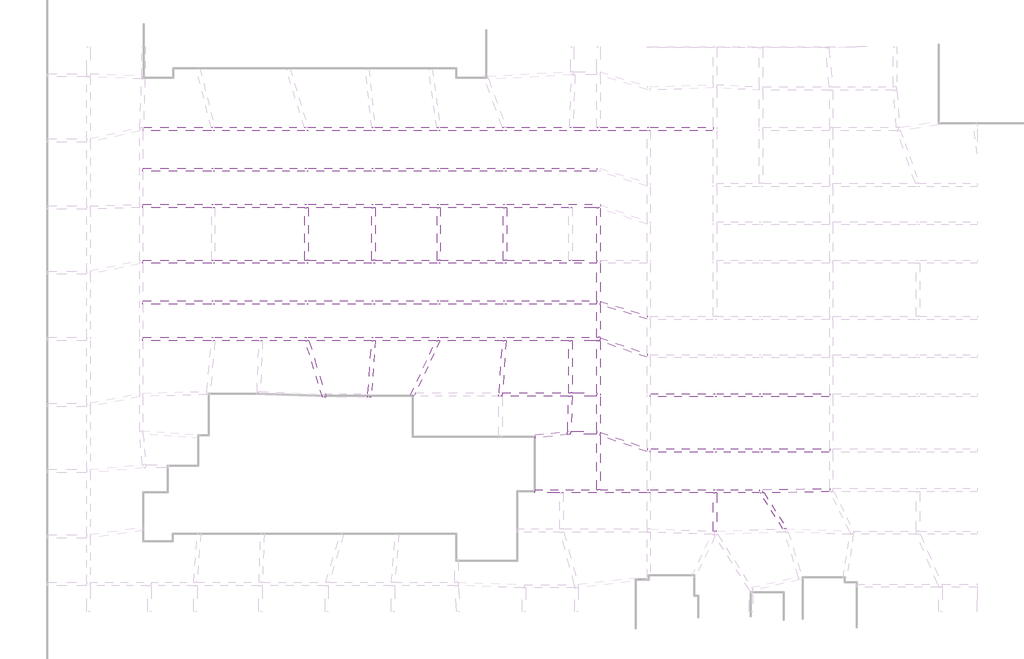
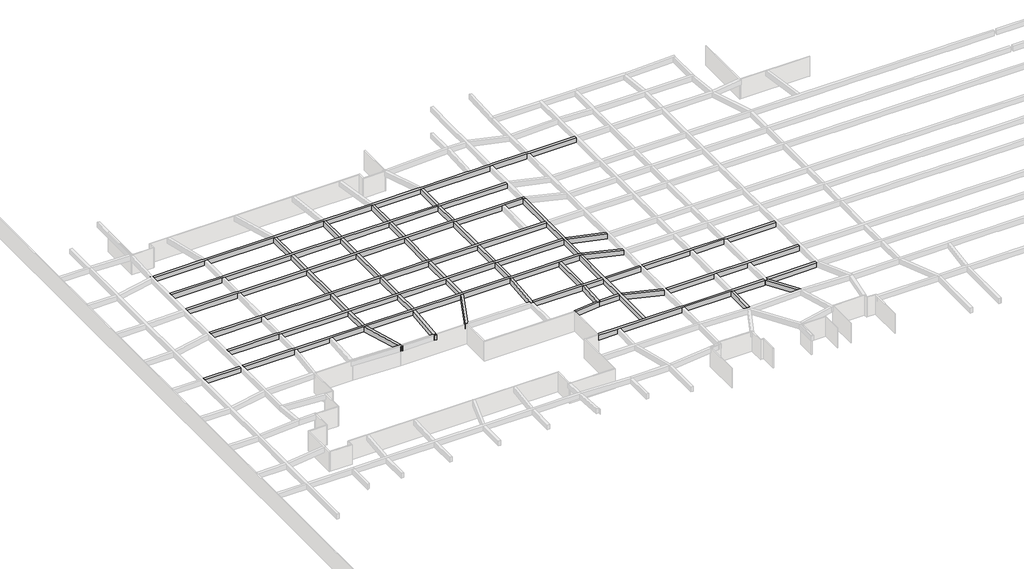
# One storey, part 31 of 45: 30 beams.
"""IFC4 building model written with IfcOpenShell, lengths in millimetres."""

from ifc_helpers import new_model, si_unit, frame, origin, place, context, project, spatial, polyline, outline, extrude, faceted_brep, element, save

model = new_model("IFC4")

# Units and contexts
model_context = context("Model", 3, world=origin())
ifc_project = project(units=[si_unit("LENGTHUNIT", "METRE", prefix="MILLI")], contexts=[model_context])

# Site, building, storey
site = spatial("IfcSite", under=ifc_project)
building = spatial("IfcBuilding", under=site)
storey = spatial("IfcBuildingStorey", under=building, Name="户型图", Elevation=0.0)

# Beams
placement = place(None, origin())
element("IfcBeam", 1, ObjectType="混凝土 - 矩形梁 : KL_beam", at=placement, inside=storey, context=model_context, shape_type="Brep", body=[
    faceted_brep([(-144086.9200457, 126261.1631403, 3300.0), (-144133.590805, 126250.9688143, 3300.0), (-144087.2760394, 126250.9688143, 3300.0), (-144133.590805, 126250.9688143, 2500.0), (-144086.9200457, 126261.1631403, 2500.0), (-144087.2760394, 126250.9688143, 2500.0)], [[[0, 1, 2]], [[3, 1, 0, 4]], [[1, 3, 5, 2]], [[0, 2, 5, 4]], [[5, 3, 4]]]),
    faceted_brep([(-143733.590805, 125889.9393475, 3300.0), (-143733.590805, 125889.9393475, 2500.0), (-135633.590805, 125889.9393475, 2500.0), (-135233.590805, 125889.9393475, 2500.0), (-124633.590805, 125889.9393475, 2500.0), (-124233.590805, 125889.9393475, 2500.0), (-116733.590805, 125889.9393475, 2500.0), (-116333.590805, 125889.9393475, 2500.0), (-109033.590805, 125889.9393475, 2500.0), (-108633.590805, 125889.9393475, 2500.0), (-101233.590805, 125889.9393475, 2500.0), (-100833.590805, 125889.9393475, 2500.0), (-90189.4148055, 125889.9393475, 2500.0), (-89789.4148055, 125889.9393475, 2500.0), (-84261.6804358, 125889.9393475, 2500.0), (-83861.6804358, 125889.9393475, 2500.0), (-76429.0040152, 125889.9393475, 2500.0), (-76429.0040152, 125889.9393475, 3300.0), (-83861.6804358, 125889.9393475, 3300.0), (-84261.6804358, 125889.9393475, 3300.0), (-89789.4148055, 125889.9393475, 3300.0), (-90189.4148055, 125889.9393475, 3300.0), (-100833.590805, 125889.9393475, 3300.0), (-101233.590805, 125889.9393475, 3300.0), (-108633.590805, 125889.9393475, 3300.0), (-109033.590805, 125889.9393475, 3300.0), (-116333.590805, 125889.9393475, 3300.0), (-116733.590805, 125889.9393475, 3300.0), (-124233.590805, 125889.9393475, 3300.0), (-124633.590805, 125889.9393475, 3300.0), (-135233.590805, 125889.9393475, 3300.0), (-135633.590805, 125889.9393475, 3300.0), (-143733.590805, 125928.9098807, 2500.0), (-143733.590805, 126001.9198071, 2500.0), (-143695.7753192, 126000.5992612, 2500.0), (-143685.6713407, 126289.9393475, 2500.0), (-135689.5791314, 126289.9393475, 2500.0), (-135277.3336797, 126289.9393475, 2500.0), (-124703.8752926, 126289.9393475, 2500.0), (-124285.59859, 126289.9393475, 2500.0), (-116755.7136598, 126289.9393475, 2500.0), (-116353.5103479, 126289.9393475, 2500.0), (-109063.6644864, 126289.9393475, 2500.0), (-108659.7334574, 126289.9393475, 2500.0), (-101319.2216246, 126289.9393475, 2500.0), (-100893.5505156, 126289.9393475, 2500.0), (-93386.1734955, 126289.9393475, 2500.0), (-92985.9296778, 126289.9393475, 2500.0), (-90189.4148055, 126289.9393475, 2500.0), (-89789.4148055, 126289.9393475, 2500.0), (-84261.6804358, 126289.9393475, 2500.0), (-83861.6804358, 126289.9393475, 2500.0), (-76429.0040152, 126289.9393475, 2500.0), (-143685.6713407, 126289.9393475, 3300.0), (-135689.5791314, 126289.9393475, 3300.0), (-135277.3336797, 126289.9393475, 3300.0), (-124703.8752926, 126289.9393475, 3300.0), (-124285.59859, 126289.9393475, 3300.0), (-116755.7136598, 126289.9393475, 3300.0), (-116353.5103479, 126289.9393475, 3300.0), (-109063.6644864, 126289.9393475, 3300.0), (-108659.7334574, 126289.9393475, 3300.0), (-101319.2216246, 126289.9393475, 3300.0), (-100893.5505156, 126289.9393475, 3300.0), (-93386.1734955, 126289.9393475, 3300.0), (-92985.9296778, 126289.9393475, 3300.0), (-90189.4148055, 126289.9393475, 3300.0), (-89789.4148055, 126289.9393475, 3300.0), (-84261.6804358, 126289.9393475, 3300.0), (-83861.6804358, 126289.9393475, 3300.0), (-76429.0040152, 126289.9393475, 3300.0), (-143733.590805, 125928.9098807, 3300.0), (-143733.590805, 126001.9198071, 3300.0), (-143695.7753192, 126000.5992612, 3300.0)], [[[0, 1, 2, 3, 4, 5, 6, 7, 8, 9, 10, 11, 12, 13, 14, 15, 16, 17, 18, 19, 20, 21, 22, 23, 24, 25, 26, 27, 28, 29, 30, 31]], [[1, 32, 33, 34, 35, 36, 37, 38, 39, 40, 41, 42, 43, 44, 45, 46, 47, 48, 49, 50, 51, 52, 16, 15, 14, 13, 12, 11, 10, 9, 8, 7, 6, 5, 4, 3, 2]], [[35, 53, 54, 55, 56, 57, 58, 59, 60, 61, 62, 63, 64, 65, 66, 67, 68, 69, 70, 52, 51, 50, 49, 48, 47, 46, 45, 44, 43, 42, 41, 40, 39, 38, 37, 36]], [[1, 0, 71, 72, 33, 32]], [[73, 34, 33, 72]], [[34, 73, 53, 35]], [[71, 0, 31, 30, 29, 28, 27, 26, 25, 24, 23, 22, 21, 20, 19, 18, 17, 70, 69, 68, 67, 66, 65, 64, 63, 62, 61, 60, 59, 58, 57, 56, 55, 54, 53, 73, 72]], [[17, 16, 52, 70]]]),
])
element("IfcBeam", 2, ObjectType="混凝土 - 矩形梁 : KL_beam", at=placement, inside=storey, context=model_context, shape_type="Brep", body=[
    faceted_brep([(-143733.590805, 121489.9393475, 3300.0), (-143733.590805, 121089.9393475, 3300.0), (-135633.590805, 121089.9393475, 3300.0), (-135233.590805, 121089.9393475, 3300.0), (-124633.590805, 121089.9393475, 3300.0), (-124233.590805, 121089.9393475, 3300.0), (-116733.590805, 121089.9393475, 3300.0), (-116333.590805, 121089.9393475, 3300.0), (-109033.590805, 121089.9393475, 3300.0), (-108633.590805, 121089.9393475, 3300.0), (-101233.590805, 121089.9393475, 3300.0), (-100833.590805, 121089.9393475, 3300.0), (-90189.4148055, 121089.9393475, 3300.0), (-90189.4148055, 121489.9393475, 3300.0), (-100833.590805, 121489.9393475, 3300.0), (-101233.590805, 121489.9393475, 3300.0), (-108633.590805, 121489.9393475, 3300.0), (-109033.590805, 121489.9393475, 3300.0), (-116333.590805, 121489.9393475, 3300.0), (-116733.590805, 121489.9393475, 3300.0), (-124233.590805, 121489.9393475, 3300.0), (-124633.590805, 121489.9393475, 3300.0), (-135233.590805, 121489.9393475, 3300.0), (-135633.590805, 121489.9393475, 3300.0), (-143733.590805, 121089.9393475, 2500.0), (-135633.590805, 121089.9393475, 2500.0), (-135233.590805, 121089.9393475, 2500.0), (-124633.590805, 121089.9393475, 2500.0), (-124233.590805, 121089.9393475, 2500.0), (-116733.590805, 121089.9393475, 2500.0), (-116333.590805, 121089.9393475, 2500.0), (-109033.590805, 121089.9393475, 2500.0), (-108633.590805, 121089.9393475, 2500.0), (-101233.590805, 121089.9393475, 2500.0), (-100833.590805, 121089.9393475, 2500.0), (-90189.4148055, 121089.9393475, 2500.0), (-143733.590805, 121489.9393475, 2500.0), (-135633.590805, 121489.9393475, 2500.0), (-135233.590805, 121489.9393475, 2500.0), (-124633.590805, 121489.9393475, 2500.0), (-124233.590805, 121489.9393475, 2500.0), (-116733.590805, 121489.9393475, 2500.0), (-116333.590805, 121489.9393475, 2500.0), (-109033.590805, 121489.9393475, 2500.0), (-108633.590805, 121489.9393475, 2500.0), (-101233.590805, 121489.9393475, 2500.0), (-100833.590805, 121489.9393475, 2500.0), (-90189.4148055, 121489.9393475, 2500.0)], [[[0, 1, 2, 3, 4, 5, 6, 7, 8, 9, 10, 11, 12, 13, 14, 15, 16, 17, 18, 19, 20, 21, 22, 23]], [[1, 24, 25, 26, 27, 28, 29, 30, 31, 32, 33, 34, 35, 12, 11, 10, 9, 8, 7, 6, 5, 4, 3, 2]], [[24, 36, 37, 38, 39, 40, 41, 42, 43, 44, 45, 46, 47, 35, 34, 33, 32, 31, 30, 29, 28, 27, 26, 25]], [[36, 0, 23, 22, 21, 20, 19, 18, 17, 16, 15, 14, 13, 47, 46, 45, 44, 43, 42, 41, 40, 39, 38, 37]], [[1, 0, 36, 24]], [[13, 12, 35, 47]]]),
])
element("IfcBeam", 3, ObjectType="混凝土 - 矩形梁 : KL_beam", at=placement, inside=storey, context=model_context, shape_type="Brep", body=[
    faceted_brep([(-89789.238806, 116812.9362228, 3300.0), (-89789.238806, 117155.5342348, 3300.0), (-89789.238806, 117212.9362228, 3300.0), (-100833.590805, 117212.9362228, 3300.0), (-101233.590805, 117212.9362228, 3300.0), (-108633.590805, 117212.9362228, 3300.0), (-109033.590805, 117212.9362228, 3300.0), (-116333.590805, 117212.9362228, 3300.0), (-116733.590805, 117212.9362228, 3300.0), (-124233.590805, 117212.9362228, 3300.0), (-124633.590805, 117212.9362228, 3300.0), (-135233.590805, 117212.9362228, 3300.0), (-135633.590805, 117212.9362228, 3300.0), (-143733.590805, 117212.9362228, 3300.0), (-143733.590805, 116812.9362228, 3300.0), (-135633.590805, 116812.9362228, 3300.0), (-135233.590805, 116812.9362228, 3300.0), (-124633.590805, 116812.9362228, 3300.0), (-124233.590805, 116812.9362228, 3300.0), (-116733.590805, 116812.9362228, 3300.0), (-116333.590805, 116812.9362228, 3300.0), (-109033.590805, 116812.9362228, 3300.0), (-108633.590805, 116812.9362228, 3300.0), (-101233.590805, 116812.9362228, 3300.0), (-100833.590805, 116812.9362228, 3300.0), (-93489.238806, 116812.9362228, 3300.0), (-93089.238806, 116812.9362228, 3300.0), (-90189.238806, 116812.9362228, 3300.0), (-89789.238806, 117212.9362228, 2500.0), (-100833.590805, 117212.9362228, 2500.0), (-101233.590805, 117212.9362228, 2500.0), (-108633.590805, 117212.9362228, 2500.0), (-109033.590805, 117212.9362228, 2500.0), (-116333.590805, 117212.9362228, 2500.0), (-116733.590805, 117212.9362228, 2500.0), (-124233.590805, 117212.9362228, 2500.0), (-124633.590805, 117212.9362228, 2500.0), (-135233.590805, 117212.9362228, 2500.0), (-135633.590805, 117212.9362228, 2500.0), (-143733.590805, 117212.9362228, 2500.0), (-89789.238806, 117155.5342348, 2500.0), (-89789.238806, 116812.9362228, 2500.0), (-90189.238806, 116812.9362228, 2500.0), (-93089.238806, 116812.9362228, 2500.0), (-93489.238806, 116812.9362228, 2500.0), (-100833.590805, 116812.9362228, 2500.0), (-101233.590805, 116812.9362228, 2500.0), (-108633.590805, 116812.9362228, 2500.0), (-109033.590805, 116812.9362228, 2500.0), (-116333.590805, 116812.9362228, 2500.0), (-116733.590805, 116812.9362228, 2500.0), (-124233.590805, 116812.9362228, 2500.0), (-124633.590805, 116812.9362228, 2500.0), (-135233.590805, 116812.9362228, 2500.0), (-135633.590805, 116812.9362228, 2500.0), (-143733.590805, 116812.9362228, 2500.0)], [[[0, 1, 2, 3, 4, 5, 6, 7, 8, 9, 10, 11, 12, 13, 14, 15, 16, 17, 18, 19, 20, 21, 22, 23, 24, 25, 26, 27]], [[2, 28, 29, 30, 31, 32, 33, 34, 35, 36, 37, 38, 39, 13, 12, 11, 10, 9, 8, 7, 6, 5, 4, 3]], [[28, 40, 41, 42, 43, 44, 45, 46, 47, 48, 49, 50, 51, 52, 53, 54, 55, 39, 38, 37, 36, 35, 34, 33, 32, 31, 30, 29]], [[41, 0, 27, 26, 25, 24, 23, 22, 21, 20, 19, 18, 17, 16, 15, 14, 55, 54, 53, 52, 51, 50, 49, 48, 47, 46, 45, 44, 43, 42]], [[14, 13, 39, 55]], [[2, 1, 0, 41, 40, 28]]]),
])
element("IfcBeam", 4, ObjectType="混凝土 - 矩形梁 : KL_beam", at=placement, inside=storey, context=model_context, shape_type="Brep", body=[
    faceted_brep([(-143733.590805, 110629.932653, 3300.0), (-143733.590805, 110229.932653, 3300.0), (-135633.590805, 110229.932653, 3300.0), (-135233.590805, 110229.932653, 3300.0), (-124633.590805, 110229.932653, 3300.0), (-124233.590805, 110229.932653, 3300.0), (-116733.590805, 110229.932653, 3300.0), (-116333.590805, 110229.932653, 3300.0), (-109033.590805, 110229.932653, 3300.0), (-108633.590805, 110229.932653, 3300.0), (-101233.590805, 110229.932653, 3300.0), (-100833.590805, 110229.932653, 3300.0), (-90189.238806, 110229.932653, 3300.0), (-90189.238806, 110629.932653, 3300.0), (-93089.238806, 110629.932653, 3300.0), (-93489.238806, 110629.932653, 3300.0), (-100833.590805, 110629.932653, 3300.0), (-101233.590805, 110629.932653, 3300.0), (-108633.590805, 110629.932653, 3300.0), (-109033.590805, 110629.932653, 3300.0), (-116333.590805, 110629.932653, 3300.0), (-116733.590805, 110629.932653, 3300.0), (-124233.590805, 110629.932653, 3300.0), (-124633.590805, 110629.932653, 3300.0), (-135233.590805, 110629.932653, 3300.0), (-135633.590805, 110629.932653, 3300.0), (-143733.590805, 110229.932653, 2500.0), (-135633.590805, 110229.932653, 2500.0), (-135233.590805, 110229.932653, 2500.0), (-124633.590805, 110229.932653, 2500.0), (-124233.590805, 110229.932653, 2500.0), (-116733.590805, 110229.932653, 2500.0), (-116333.590805, 110229.932653, 2500.0), (-109033.590805, 110229.932653, 2500.0), (-108633.590805, 110229.932653, 2500.0), (-101233.590805, 110229.932653, 2500.0), (-100833.590805, 110229.932653, 2500.0), (-90189.238806, 110229.932653, 2500.0), (-143733.590805, 110629.932653, 2500.0), (-135633.590805, 110629.932653, 2500.0), (-135233.590805, 110629.932653, 2500.0), (-124633.590805, 110629.932653, 2500.0), (-124233.590805, 110629.932653, 2500.0), (-116733.590805, 110629.932653, 2500.0), (-116333.590805, 110629.932653, 2500.0), (-109033.590805, 110629.932653, 2500.0), (-108633.590805, 110629.932653, 2500.0), (-101233.590805, 110629.932653, 2500.0), (-100833.590805, 110629.932653, 2500.0), (-93489.238806, 110629.932653, 2500.0), (-93089.238806, 110629.932653, 2500.0), (-90189.238806, 110629.932653, 2500.0)], [[[0, 1, 2, 3, 4, 5, 6, 7, 8, 9, 10, 11, 12, 13, 14, 15, 16, 17, 18, 19, 20, 21, 22, 23, 24, 25]], [[1, 26, 27, 28, 29, 30, 31, 32, 33, 34, 35, 36, 37, 12, 11, 10, 9, 8, 7, 6, 5, 4, 3, 2]], [[26, 38, 39, 40, 41, 42, 43, 44, 45, 46, 47, 48, 49, 50, 51, 37, 36, 35, 34, 33, 32, 31, 30, 29, 28, 27]], [[38, 0, 25, 24, 23, 22, 21, 20, 19, 18, 17, 16, 15, 14, 13, 51, 50, 49, 48, 47, 46, 45, 44, 43, 42, 41, 40, 39]], [[1, 0, 38, 26]], [[13, 12, 37, 51]]]),
])
element("IfcBeam", 5, ObjectType="混凝土 - 矩形梁 : KL_beam", at=placement, inside=storey, context=model_context, shape_type="Brep", body=[
    faceted_brep([(-143733.590805, 105823.4823743, 3300.0), (-143733.590805, 105423.4823743, 3300.0), (-135633.590805, 105423.4823743, 3300.0), (-135233.590805, 105423.4823743, 3300.0), (-124633.590805, 105423.4823743, 3300.0), (-124233.590805, 105423.4823743, 3300.0), (-116733.590805, 105423.4823743, 3300.0), (-116333.590805, 105423.4823743, 3300.0), (-109033.590805, 105423.4823743, 3300.0), (-108633.590805, 105423.4823743, 3300.0), (-101233.590805, 105423.4823743, 3300.0), (-100833.590805, 105423.4823743, 3300.0), (-90189.238806, 105423.4823743, 3300.0), (-90189.238806, 105823.4823743, 3300.0), (-100833.590805, 105823.4823743, 3300.0), (-101233.590805, 105823.4823743, 3300.0), (-108633.590805, 105823.4823743, 3300.0), (-109033.590805, 105823.4823743, 3300.0), (-116333.590805, 105823.4823743, 3300.0), (-116733.590805, 105823.4823743, 3300.0), (-124233.590805, 105823.4823743, 3300.0), (-124633.590805, 105823.4823743, 3300.0), (-135233.590805, 105823.4823743, 3300.0), (-135633.590805, 105823.4823743, 3300.0), (-143733.590805, 105823.4823743, 2500.0), (-90189.238806, 105823.4823743, 2500.0), (-100833.590805, 105823.4823743, 2500.0), (-101233.590805, 105823.4823743, 2500.0), (-108633.590805, 105823.4823743, 2500.0), (-109033.590805, 105823.4823743, 2500.0), (-116333.590805, 105823.4823743, 2500.0), (-116733.590805, 105823.4823743, 2500.0), (-124233.590805, 105823.4823743, 2500.0), (-124633.590805, 105823.4823743, 2500.0), (-135233.590805, 105823.4823743, 2500.0), (-135633.590805, 105823.4823743, 2500.0), (-143733.590805, 105423.4823743, 2500.0), (-90189.238806, 105423.4823743, 2500.0), (-100833.590805, 105423.4823743, 2500.0), (-101233.590805, 105423.4823743, 2500.0), (-108633.590805, 105423.4823743, 2500.0), (-109033.590805, 105423.4823743, 2500.0), (-116333.590805, 105423.4823743, 2500.0), (-116733.590805, 105423.4823743, 2500.0), (-124233.590805, 105423.4823743, 2500.0), (-124633.590805, 105423.4823743, 2500.0), (-135233.590805, 105423.4823743, 2500.0), (-135633.590805, 105423.4823743, 2500.0)], [[[0, 1, 2, 3, 4, 5, 6, 7, 8, 9, 10, 11, 12, 13, 14, 15, 16, 17, 18, 19, 20, 21, 22, 23]], [[24, 0, 23, 22, 21, 20, 19, 18, 17, 16, 15, 14, 13, 25, 26, 27, 28, 29, 30, 31, 32, 33, 34, 35]], [[36, 24, 35, 34, 33, 32, 31, 30, 29, 28, 27, 26, 25, 37, 38, 39, 40, 41, 42, 43, 44, 45, 46, 47]], [[1, 36, 47, 46, 45, 44, 43, 42, 41, 40, 39, 38, 37, 12, 11, 10, 9, 8, 7, 6, 5, 4, 3, 2]], [[1, 0, 24, 36]], [[13, 12, 37, 25]]]),
])
element("IfcBeam", 6, ObjectType="混凝土 - 矩形梁 : KL_beam", at=placement, inside=storey, context=model_context, shape_type="Brep", body=[
    faceted_brep([(-89789.238806, 101129.932653, 3300.0), (-89789.238806, 101472.4855519, 3300.0), (-89789.238806, 101529.932653, 3300.0), (-90189.238806, 101529.932653, 3300.0), (-100833.590805, 101529.932653, 3300.0), (-101233.590805, 101529.932653, 3300.0), (-108633.590805, 101529.932653, 3300.0), (-109033.590805, 101529.932653, 3300.0), (-116333.590805, 101529.932653, 3300.0), (-116733.590805, 101529.932653, 3300.0), (-124233.590805, 101529.932653, 3300.0), (-124633.590805, 101529.932653, 3300.0), (-135233.590805, 101529.932653, 3300.0), (-135633.590805, 101529.932653, 3300.0), (-143733.590805, 101529.932653, 3300.0), (-143733.590805, 101129.932653, 3300.0), (-135651.8525052, 101129.932653, 3300.0), (-135250.3245702, 101129.932653, 3300.0), (-130040.6968677, 101129.932653, 3300.0), (-129640.45305, 101129.932653, 3300.0), (-124581.5819966, 101129.932653, 3300.0), (-124163.305294, 101129.932653, 3300.0), (-116748.064547, 101129.932653, 3300.0), (-116347.0877878, 101129.932653, 3300.0), (-109147.5279204, 101129.932653, 3300.0), (-108706.1767528, 101129.932653, 3300.0), (-101293.6262259, 101129.932653, 3300.0), (-100892.6494666, 101129.932653, 3300.0), (-93489.8138642, 101129.932653, 3300.0), (-93089.8138642, 101129.932653, 3300.0), (-90189.8138642, 101129.932653, 3300.0), (-90023.0143455, 101129.932653, 3300.0), (-89789.238806, 101129.932653, 2500.0), (-143733.590805, 101129.932653, 2500.0), (-135651.8525052, 101129.932653, 2500.0), (-135250.3245702, 101129.932653, 2500.0), (-130040.6968677, 101129.932653, 2500.0), (-129640.45305, 101129.932653, 2500.0), (-124581.5819966, 101129.932653, 2500.0), (-124163.305294, 101129.932653, 2500.0), (-116748.064547, 101129.932653, 2500.0), (-116347.0877878, 101129.932653, 2500.0), (-109147.5279204, 101129.932653, 2500.0), (-108706.1767528, 101129.932653, 2500.0), (-101293.6262259, 101129.932653, 2500.0), (-100892.6494666, 101129.932653, 2500.0), (-93489.8138642, 101129.932653, 2500.0), (-93089.8138642, 101129.932653, 2500.0), (-90189.8138642, 101129.932653, 2500.0), (-90023.0143455, 101129.932653, 2500.0), (-89789.238806, 101529.932653, 2500.0), (-89789.238806, 101472.4855519, 2500.0), (-143733.590805, 101529.932653, 2500.0), (-135633.590805, 101529.932653, 2500.0), (-135233.590805, 101529.932653, 2500.0), (-124633.590805, 101529.932653, 2500.0), (-124233.590805, 101529.932653, 2500.0), (-116733.590805, 101529.932653, 2500.0), (-116333.590805, 101529.932653, 2500.0), (-109033.590805, 101529.932653, 2500.0), (-108633.590805, 101529.932653, 2500.0), (-101233.590805, 101529.932653, 2500.0), (-100833.590805, 101529.932653, 2500.0), (-90189.238806, 101529.932653, 2500.0)], [[[0, 1, 2, 3, 4, 5, 6, 7, 8, 9, 10, 11, 12, 13, 14, 15, 16, 17, 18, 19, 20, 21, 22, 23, 24, 25, 26, 27, 28, 29, 30, 31]], [[32, 0, 31, 30, 29, 28, 27, 26, 25, 24, 23, 22, 21, 20, 19, 18, 17, 16, 15, 33, 34, 35, 36, 37, 38, 39, 40, 41, 42, 43, 44, 45, 46, 47, 48, 49]], [[50, 51, 32, 49, 48, 47, 46, 45, 44, 43, 42, 41, 40, 39, 38, 37, 36, 35, 34, 33, 52, 53, 54, 55, 56, 57, 58, 59, 60, 61, 62, 63]], [[2, 50, 63, 62, 61, 60, 59, 58, 57, 56, 55, 54, 53, 52, 14, 13, 12, 11, 10, 9, 8, 7, 6, 5, 4, 3]], [[15, 14, 52, 33]], [[2, 1, 0, 32, 51, 50]]]),
    faceted_brep([(-149959.8528414, 101129.932653, 3300.0), (-149959.8528414, 101529.932653, 3300.0), (-149959.8528414, 101529.932653, 2500.0), (-149959.8528414, 101129.932653, 2500.0), (-144133.590805, 101529.932653, 3300.0), (-144133.590805, 101129.932653, 3300.0), (-144133.590805, 101129.932653, 2500.0), (-144133.590805, 101529.932653, 2500.0)], [[[0, 1, 2, 3]], [[4, 5, 6, 7]], [[1, 0, 5, 4]], [[0, 3, 6, 5]], [[3, 2, 7, 6]], [[2, 1, 4, 7]]]),
])
element("IfcBeam", 7, ObjectType="混凝土 - 矩形梁 : KL_beam", at=placement, inside=storey, context=model_context, shape_type="SweptSolid", body=[
    extrude(outline(polyline([(-124633.590805, 125889.9393475), (-124233.590805, 125889.9393475), (-124233.590805, 121489.9393475), (-124633.590805, 121489.9393475), (-124633.590805, 125889.9393475)])), frame((0.0, 0.0, 2500.0), z_axis=(0.0, 0.0, 1.0), x_axis=(1.0, 0.0, 0.0)), (0.0, 0.0, 1.0), 800.0),
    extrude(outline(polyline([(-124233.590805, 101529.932653), (-124633.590805, 101529.932653), (-124633.590805, 105423.4823743), (-124233.590805, 105423.4823743), (-124233.590805, 101529.932653)])), frame((0.0, 0.0, 2500.0), z_axis=(0.0, 0.0, 1.0), x_axis=(1.0, 0.0, 0.0)), (0.0, 0.0, 1.0), 800.0),
    extrude(outline(polyline([(-124633.590805, 121089.9393475), (-124233.590805, 121089.9393475), (-124233.590805, 117212.9362228), (-124633.590805, 117212.9362228), (-124633.590805, 121089.9393475)])), frame((0.0, 0.0, 2500.0), z_axis=(0.0, 0.0, 1.0), x_axis=(1.0, 0.0, 0.0)), (0.0, 0.0, 1.0), 800.0),
    extrude(outline(polyline([(-124633.590805, 116812.9362228), (-124233.590805, 116812.9362228), (-124233.590805, 110629.932653), (-124633.590805, 110629.932653), (-124633.590805, 116812.9362228)])), frame((0.0, 0.0, 2500.0), z_axis=(0.0, 0.0, 1.0), x_axis=(1.0, 0.0, 0.0)), (0.0, 0.0, 1.0), 800.0),
    extrude(outline(polyline([(-124633.590805, 110229.932653), (-124233.590805, 110229.932653), (-124233.590805, 105823.4823743), (-124633.590805, 105823.4823743), (-124633.590805, 110229.932653)])), frame((0.0, 0.0, 2500.0), z_axis=(0.0, 0.0, 1.0), x_axis=(1.0, 0.0, 0.0)), (0.0, 0.0, 1.0), 800.0),
])
element("IfcBeam", 8, ObjectType="混凝土 - 矩形梁 : KL_beam", at=placement, inside=storey, context=model_context, shape_type="SweptSolid", body=[
    extrude(outline(polyline([(-116733.590805, 125889.9393475), (-116333.590805, 125889.9393475), (-116333.590805, 121489.9393475), (-116733.590805, 121489.9393475), (-116733.590805, 125889.9393475)])), frame((0.0, 0.0, 2500.0), z_axis=(0.0, 0.0, 1.0), x_axis=(1.0, 0.0, 0.0)), (0.0, 0.0, 1.0), 800.0),
    extrude(outline(polyline([(-116333.590805, 101529.932653), (-116733.590805, 101529.932653), (-116733.590805, 105423.4823743), (-116333.590805, 105423.4823743), (-116333.590805, 101529.932653)])), frame((0.0, 0.0, 2500.0), z_axis=(0.0, 0.0, 1.0), x_axis=(1.0, 0.0, 0.0)), (0.0, 0.0, 1.0), 800.0),
    extrude(outline(polyline([(-116733.590805, 121089.9393475), (-116333.590805, 121089.9393475), (-116333.590805, 117212.9362228), (-116733.590805, 117212.9362228), (-116733.590805, 121089.9393475)])), frame((0.0, 0.0, 2500.0), z_axis=(0.0, 0.0, 1.0), x_axis=(1.0, 0.0, 0.0)), (0.0, 0.0, 1.0), 800.0),
    extrude(outline(polyline([(-116733.590805, 116812.9362228), (-116333.590805, 116812.9362228), (-116333.590805, 110629.932653), (-116733.590805, 110629.932653), (-116733.590805, 116812.9362228)])), frame((0.0, 0.0, 2500.0), z_axis=(0.0, 0.0, 1.0), x_axis=(1.0, 0.0, 0.0)), (0.0, 0.0, 1.0), 800.0),
    extrude(outline(polyline([(-116733.590805, 110229.932653), (-116333.590805, 110229.932653), (-116333.590805, 105823.4823743), (-116733.590805, 105823.4823743), (-116733.590805, 110229.932653)])), frame((0.0, 0.0, 2500.0), z_axis=(0.0, 0.0, 1.0), x_axis=(1.0, 0.0, 0.0)), (0.0, 0.0, 1.0), 800.0),
])
element("IfcBeam", 9, ObjectType="混凝土 - 矩形梁 : KL_beam", at=placement, inside=storey, context=model_context, shape_type="SweptSolid", body=[
    extrude(outline(polyline([(-109033.590805, 125889.9393475), (-108633.590805, 125889.9393475), (-108633.590805, 121489.9393475), (-109033.590805, 121489.9393475), (-109033.590805, 125889.9393475)])), frame((0.0, 0.0, 2500.0), z_axis=(0.0, 0.0, 1.0), x_axis=(1.0, 0.0, 0.0)), (0.0, 0.0, 1.0), 800.0),
    extrude(outline(polyline([(-108633.590805, 101529.932653), (-109033.590805, 101529.932653), (-109033.590805, 105423.4823743), (-108633.590805, 105423.4823743), (-108633.590805, 101529.932653)])), frame((0.0, 0.0, 2500.0), z_axis=(0.0, 0.0, 1.0), x_axis=(1.0, 0.0, 0.0)), (0.0, 0.0, 1.0), 800.0),
    extrude(outline(polyline([(-109033.590805, 121089.9393475), (-108633.590805, 121089.9393475), (-108633.590805, 117212.9362228), (-109033.590805, 117212.9362228), (-109033.590805, 121089.9393475)])), frame((0.0, 0.0, 2500.0), z_axis=(0.0, 0.0, 1.0), x_axis=(1.0, 0.0, 0.0)), (0.0, 0.0, 1.0), 800.0),
    extrude(outline(polyline([(-109033.590805, 116812.9362228), (-108633.590805, 116812.9362228), (-108633.590805, 110629.932653), (-109033.590805, 110629.932653), (-109033.590805, 116812.9362228)])), frame((0.0, 0.0, 2500.0), z_axis=(0.0, 0.0, 1.0), x_axis=(1.0, 0.0, 0.0)), (0.0, 0.0, 1.0), 800.0),
    extrude(outline(polyline([(-109033.590805, 110229.932653), (-108633.590805, 110229.932653), (-108633.590805, 105823.4823743), (-109033.590805, 105823.4823743), (-109033.590805, 110229.932653)])), frame((0.0, 0.0, 2500.0), z_axis=(0.0, 0.0, 1.0), x_axis=(1.0, 0.0, 0.0)), (0.0, 0.0, 1.0), 800.0),
])
element("IfcBeam", 10, ObjectType="混凝土 - 矩形梁 : KL_beam", at=placement, inside=storey, context=model_context, shape_type="SweptSolid", body=[
    extrude(outline(polyline([(-101233.590805, 125889.9393475), (-100833.590805, 125889.9393475), (-100833.590805, 121489.9393475), (-101233.590805, 121489.9393475), (-101233.590805, 125889.9393475)])), frame((0.0, 0.0, 2500.0), z_axis=(0.0, 0.0, 1.0), x_axis=(1.0, 0.0, 0.0)), (0.0, 0.0, 1.0), 800.0),
    extrude(outline(polyline([(-100833.590805, 101529.932653), (-101233.590805, 101529.932653), (-101233.590805, 105423.4823743), (-100833.590805, 105423.4823743), (-100833.590805, 101529.932653)])), frame((0.0, 0.0, 2500.0), z_axis=(0.0, 0.0, 1.0), x_axis=(1.0, 0.0, 0.0)), (0.0, 0.0, 1.0), 800.0),
    extrude(outline(polyline([(-101233.590805, 121089.9393475), (-100833.590805, 121089.9393475), (-100833.590805, 117212.9362228), (-101233.590805, 117212.9362228), (-101233.590805, 121089.9393475)])), frame((0.0, 0.0, 2500.0), z_axis=(0.0, 0.0, 1.0), x_axis=(1.0, 0.0, 0.0)), (0.0, 0.0, 1.0), 800.0),
    extrude(outline(polyline([(-101233.590805, 116812.9362228), (-100833.590805, 116812.9362228), (-100833.590805, 110629.932653), (-101233.590805, 110629.932653), (-101233.590805, 116812.9362228)])), frame((0.0, 0.0, 2500.0), z_axis=(0.0, 0.0, 1.0), x_axis=(1.0, 0.0, 0.0)), (0.0, 0.0, 1.0), 800.0),
    extrude(outline(polyline([(-101233.590805, 110229.932653), (-100833.590805, 110229.932653), (-100833.590805, 105823.4823743), (-101233.590805, 105823.4823743), (-101233.590805, 110229.932653)])), frame((0.0, 0.0, 2500.0), z_axis=(0.0, 0.0, 1.0), x_axis=(1.0, 0.0, 0.0)), (0.0, 0.0, 1.0), 800.0),
])
element("IfcBeam", 11, ObjectType="混凝土 - 矩形梁 : KL_beam", at=placement, inside=storey, context=model_context, shape_type="Brep", body=[
    faceted_brep([(-89789.238806, 116812.9362228, 3300.0), (-90189.238806, 116812.9362228, 3300.0), (-90189.238806, 110629.932653, 3300.0), (-90189.238806, 110229.932653, 3300.0), (-90189.238806, 105823.4823743, 3300.0), (-90189.238806, 105423.4823743, 3300.0), (-90189.238806, 101529.932653, 3300.0), (-89789.238806, 101529.932653, 3300.0), (-89789.238806, 105353.1978867, 3300.0), (-89789.238806, 105771.4745893, 3300.0), (-89789.238806, 110229.932653, 3300.0), (-89789.238806, 110629.932653, 3300.0), (-89789.238806, 116732.4859624, 3300.0), (-90189.238806, 116812.9362228, 2500.0), (-90189.238806, 110629.932653, 2500.0), (-90189.238806, 110229.932653, 2500.0), (-90189.238806, 105823.4823743, 2500.0), (-90189.238806, 105423.4823743, 2500.0), (-90189.238806, 101529.932653, 2500.0), (-89789.238806, 116812.9362228, 2500.0), (-89789.238806, 116732.4859624, 2500.0), (-89789.238806, 110629.932653, 2500.0), (-89789.238806, 110229.932653, 2500.0), (-89789.238806, 105771.4745893, 2500.0), (-89789.238806, 105353.1978867, 2500.0), (-89789.238806, 101529.932653, 2500.0)], [[[0, 1, 2, 3, 4, 5, 6, 7, 8, 9, 10, 11, 12]], [[1, 13, 14, 15, 16, 17, 18, 6, 5, 4, 3, 2]], [[13, 19, 20, 21, 22, 23, 24, 25, 18, 17, 16, 15, 14]], [[19, 0, 12, 11, 10, 9, 8, 7, 25, 24, 23, 22, 21, 20]], [[1, 0, 19, 13]], [[7, 6, 18, 25]]]),
])
element("IfcBeam", 12, ObjectType="混凝土 - 矩形梁 : KL_beam", at=placement, inside=storey, context=model_context, shape_type="SweptSolid", body=[
    extrude(outline(polyline([(-89789.238806, 105353.1978867), (-89789.238806, 105771.4745893), (-84261.6804358, 104081.530402), (-84261.6804358, 103663.2536994), (-89789.238806, 105353.1978867)])), frame((0.0, 0.0, 2500.0), z_axis=(0.0, 0.0, 1.0), x_axis=(1.0, 0.0, 0.0)), (0.0, 0.0, 1.0), 800.0),
])
element("IfcBeam", 13, ObjectType="混凝土 - 矩形梁 : KL_beam", at=placement, inside=storey, context=model_context, shape_type="Brep", body=[
    faceted_brep([(-84261.6804358, 99146.1462985, 3300.0), (-84261.6804358, 99569.194571, 3300.0), (-89789.238806, 101472.4855519, 3300.0), (-89789.238806, 101129.932653, 3300.0), (-90023.0143455, 101129.932653, 3300.0), (-89789.8138642, 101049.6352878, 3300.0), (-84261.6804358, 99146.1462985, 2500.0), (-90023.0143455, 101129.932653, 2500.0), (-89789.8138642, 101049.6352878, 2500.0), (-84261.6804358, 99569.194571, 2500.0), (-89789.238806, 101129.932653, 2500.0), (-89789.238806, 101472.4855519, 2500.0)], [[[0, 1, 2, 3, 4, 5]], [[6, 0, 5, 4, 7, 8]], [[9, 6, 8, 7, 10, 11]], [[1, 9, 11, 2]], [[1, 0, 6, 9]], [[3, 10, 7, 4]], [[10, 3, 2, 11]]]),
])
element("IfcBeam", 14, ObjectType="混凝土 - 矩形梁 : KL_beam", at=placement, inside=storey, context=model_context, shape_type="Brep", body=[
    faceted_brep([(-90023.0143455, 101129.932653, 3300.0), (-90189.8138642, 101129.932653, 3300.0), (-90189.8138642, 94959.0757309, 3300.0), (-90189.8138642, 94559.0757309, 3300.0), (-90189.8138642, 90461.8170093, 3300.0), (-90189.8138642, 90061.8170093, 3300.0), (-90189.8138642, 83554.2865852, 3300.0), (-89789.8138642, 83554.2865852, 3300.0), (-89789.8138642, 89908.3229594, 3300.0), (-89789.8138642, 90331.3712319, 3300.0), (-89789.8138642, 94488.7126183, 3300.0), (-89789.8138642, 94888.7126183, 3300.0), (-89789.8138642, 101049.6352878, 3300.0), (-90189.8138642, 101129.932653, 2500.0), (-90189.8138642, 94959.0757309, 2500.0), (-90189.8138642, 94559.0757309, 2500.0), (-90189.8138642, 90461.8170093, 2500.0), (-90189.8138642, 90061.8170093, 2500.0), (-90189.8138642, 83554.2865852, 2500.0), (-90023.0143455, 101129.932653, 2500.0), (-89789.8138642, 101049.6352878, 2500.0), (-89789.8138642, 94888.7126183, 2500.0), (-89789.8138642, 94488.7126183, 2500.0), (-89789.8138642, 90331.3712319, 2500.0), (-89789.8138642, 89908.3229594, 2500.0), (-89789.8138642, 83554.2865852, 2500.0)], [[[0, 1, 2, 3, 4, 5, 6, 7, 8, 9, 10, 11, 12]], [[1, 13, 14, 15, 16, 17, 18, 6, 5, 4, 3, 2]], [[13, 19, 20, 21, 22, 23, 24, 25, 18, 17, 16, 15, 14]], [[20, 12, 11, 10, 9, 8, 7, 25, 24, 23, 22, 21]], [[13, 1, 0, 19]], [[0, 12, 20, 19]], [[7, 6, 18, 25]]]),
])
element("IfcBeam", 15, ObjectType="混凝土 - 矩形梁 : KL_beam", at=placement, inside=storey, context=model_context, shape_type="Brep", body=[
    faceted_brep([(-89789.8138642, 94888.7126183, 3300.0), (-89789.8138642, 94488.7126183, 3300.0), (-84261.6804358, 94488.7126183, 3300.0), (-84261.6804358, 94888.7126183, 3300.0), (-89789.8138642, 94488.7126183, 2500.0), (-84261.6804358, 94488.7126183, 2500.0), (-89789.8138642, 94888.7126183, 2500.0), (-84261.6804358, 94888.7126183, 2500.0)], [[[0, 1, 2, 3]], [[1, 4, 5, 2]], [[4, 6, 7, 5]], [[6, 0, 3, 7]], [[1, 0, 6, 4]], [[3, 2, 5, 7]]]),
    faceted_brep([(-83861.6804358, 94488.7126183, 3300.0), (-83861.6804358, 94888.7126183, 3300.0), (-83861.6804358, 94888.7126183, 2500.0), (-83861.6804358, 94488.7126183, 2500.0), (-76429.0040152, 94488.7126183, 3300.0), (-76029.0040152, 94488.7126183, 3300.0), (-71019.6378921, 94488.7126183, 3300.0), (-70619.6378921, 94488.7126183, 3300.0), (-62729.0040152, 94488.7126183, 3300.0), (-62729.0040152, 94888.7126183, 3300.0), (-70619.6378921, 94888.7126183, 3300.0), (-71019.6378921, 94888.7126183, 3300.0), (-76029.0040152, 94888.7126183, 3300.0), (-76429.0040152, 94888.7126183, 3300.0), (-76429.0040152, 94488.7126183, 2500.0), (-76029.0040152, 94488.7126183, 2500.0), (-71019.6378921, 94488.7126183, 2500.0), (-70619.6378921, 94488.7126183, 2500.0), (-62729.0040152, 94488.7126183, 2500.0), (-76429.0040152, 94888.7126183, 2500.0), (-76029.0040152, 94888.7126183, 2500.0), (-71019.6378921, 94888.7126183, 2500.0), (-70619.6378921, 94888.7126183, 2500.0), (-62729.0040152, 94888.7126183, 2500.0)], [[[0, 1, 2, 3]], [[1, 0, 4, 5, 6, 7, 8, 9, 10, 11, 12, 13]], [[0, 3, 14, 15, 16, 17, 18, 8, 7, 6, 5, 4]], [[3, 2, 19, 20, 21, 22, 23, 18, 17, 16, 15, 14]], [[2, 1, 13, 12, 11, 10, 9, 23, 22, 21, 20, 19]], [[9, 8, 18, 23]]]),
])
element("IfcBeam", 16, ObjectType="混凝土 - 矩形梁 : KL_beam", at=placement, inside=storey, context=model_context, shape_type="SweptSolid", body=[
    extrude(outline(polyline([(-84261.6804358, 88427.8822425), (-84261.6804358, 88004.83397), (-89789.8138642, 89908.3229594), (-89789.8138642, 90331.3712319), (-84261.6804358, 88427.8822425)])), frame((0.0, 0.0, 2500.0), z_axis=(0.0, 0.0, 1.0), x_axis=(1.0, 0.0, 0.0)), (0.0, 0.0, 1.0), 800.0),
])
element("IfcBeam", 17, ObjectType="混凝土 - 矩形梁 : KL_beam", at=placement, inside=storey, context=model_context, shape_type="Brep", body=[
    faceted_brep([(-83861.6804358, 88347.4925836, 3300.0), (-83861.6804358, 87947.4925836, 3300.0), (-76429.0040152, 87947.4925836, 3300.0), (-76029.0040152, 87947.4925836, 3300.0), (-71019.6378921, 87947.4925836, 3300.0), (-70619.6378921, 87947.4925836, 3300.0), (-62729.0040152, 87947.4925836, 3300.0), (-62729.0040152, 88347.4925836, 3300.0), (-70619.6378921, 88347.4925836, 3300.0), (-71019.6378921, 88347.4925836, 3300.0), (-76029.0040152, 88347.4925836, 3300.0), (-76429.0040152, 88347.4925836, 3300.0), (-83861.6804358, 87947.4925836, 2500.0), (-76429.0040152, 87947.4925836, 2500.0), (-76029.0040152, 87947.4925836, 2500.0), (-71019.6378921, 87947.4925836, 2500.0), (-70619.6378921, 87947.4925836, 2500.0), (-62729.0040152, 87947.4925836, 2500.0), (-83861.6804358, 88347.4925836, 2500.0), (-76429.0040152, 88347.4925836, 2500.0), (-76029.0040152, 88347.4925836, 2500.0), (-71019.6378921, 88347.4925836, 2500.0), (-70619.6378921, 88347.4925836, 2500.0), (-62729.0040152, 88347.4925836, 2500.0)], [[[0, 1, 2, 3, 4, 5, 6, 7, 8, 9, 10, 11]], [[1, 12, 13, 14, 15, 16, 17, 6, 5, 4, 3, 2]], [[12, 18, 19, 20, 21, 22, 23, 17, 16, 15, 14, 13]], [[18, 0, 11, 10, 9, 8, 7, 23, 22, 21, 20, 19]], [[1, 0, 18, 12]], [[7, 6, 17, 23]]]),
])
element("IfcBeam", 18, ObjectType="混凝土 - 矩形梁 : KL_beam", at=placement, inside=storey, context=model_context, shape_type="Brep", body=[
    faceted_brep([(-122538.1762195, 94446.2535162, 3300.0), (-122119.8995169, 94446.2535162, 3300.0), (-122242.1917895, 94846.2535162, 3300.0), (-124163.305294, 101129.932653, 3300.0), (-124581.5819966, 101129.932653, 3300.0), (-122538.1762195, 94446.2535162, 2500.0), (-124581.5819966, 101129.932653, 2500.0), (-122119.8995169, 94446.2535162, 2500.0), (-124163.305294, 101129.932653, 2500.0), (-122242.1917895, 94846.2535162, 2500.0)], [[[0, 1, 2, 3, 4]], [[5, 0, 4, 6]], [[7, 5, 6, 8, 9]], [[1, 7, 9, 8, 3, 2]], [[4, 3, 8, 6]], [[1, 0, 5, 7]]]),
])
element("IfcBeam", 19, ObjectType="混凝土 - 矩形梁 : KL_beam", at=placement, inside=storey, context=model_context, shape_type="Brep", body=[
    faceted_brep([(-117215.4329211, 94446.2535162, 3300.0), (-116814.4561618, 94446.2535162, 3300.0), (-116347.0877878, 101129.932653, 3300.0), (-116748.064547, 101129.932653, 3300.0), (-117187.4621963, 94846.2535162, 3300.0), (-117215.4329211, 94446.2535162, 2500.0), (-116748.064547, 101129.932653, 2500.0), (-117187.4621963, 94846.2535162, 2500.0), (-116814.4561618, 94446.2535162, 2500.0), (-116347.0877878, 101129.932653, 2500.0)], [[[0, 1, 2, 3, 4]], [[5, 0, 4, 3, 6, 7]], [[8, 5, 7, 6, 9]], [[1, 8, 9, 2]], [[3, 2, 9, 6]], [[1, 0, 5, 8]]]),
])
element("IfcBeam", 20, ObjectType="混凝土 - 矩形梁 : KL_beam", at=placement, inside=storey, context=model_context, shape_type="Brep", body=[
    faceted_brep([(-112132.6953167, 94728.2205126, 3300.0), (-111770.1722019, 94559.1732079, 3300.0), (-111583.6491387, 94959.1732079, 3300.0), (-108706.1767528, 101129.932653, 3300.0), (-109147.5279204, 101129.932653, 3300.0), (-112132.6953167, 94728.2205126, 2500.0), (-109147.5279204, 101129.932653, 2500.0), (-111770.1722019, 94559.1732079, 2500.0), (-108706.1767528, 101129.932653, 2500.0), (-111583.6491387, 94959.1732079, 2500.0)], [[[0, 1, 2, 3, 4]], [[5, 0, 4, 6]], [[7, 5, 6, 8, 9]], [[1, 7, 9, 8, 3, 2]], [[4, 3, 8, 6]], [[1, 0, 5, 7]]]),
])
element("IfcBeam", 21, ObjectType="混凝土 - 矩形梁 : KL_beam", at=placement, inside=storey, context=model_context, shape_type="Brep", body=[
    faceted_brep([(-101753.0984859, 94559.1732079, 3300.0), (-101738.6349683, 94559.1732079, 3300.0), (-101352.1217267, 94559.1732079, 3300.0), (-101324.1578182, 94959.0757309, 3300.0), (-100892.6494666, 101129.932653, 3300.0), (-101293.6262259, 101129.932653, 3300.0), (-101725.1277611, 94959.1732079, 3300.0), (-101352.1217267, 94559.1732079, 2500.0), (-101324.1578182, 94959.0757309, 2500.0), (-100892.6494666, 101129.932653, 2500.0), (-101738.6349683, 94559.1732079, 2500.0), (-101753.0984859, 94559.1732079, 2500.0), (-101725.1277611, 94959.1732079, 2500.0), (-101293.6262259, 101129.932653, 2500.0)], [[[0, 1, 2, 3, 4, 5, 6]], [[2, 7, 8, 9, 4, 3]], [[7, 10, 11, 12, 13, 9, 8]], [[11, 0, 6, 5, 13, 12]], [[5, 4, 9, 13]], [[2, 1, 0, 11, 10, 7]]]),
])
element("IfcBeam", 22, ObjectType="混凝土 - 矩形梁 : KL_beam", at=placement, inside=storey, context=model_context, shape_type="Brep", body=[
    faceted_brep([(-101324.1578182, 94959.0757309, 3300.0), (-101352.1285429, 94559.0757309, 3300.0), (-101338.6349683, 94559.0757309, 3300.0), (-93496.919927, 94559.0757309, 3300.0), (-93096.6761093, 94559.0757309, 3300.0), (-90189.8138642, 94559.0757309, 3300.0), (-90189.8138642, 94959.0757309, 3300.0), (-93089.8138642, 94959.0757309, 3300.0), (-93489.8138642, 94959.0757309, 3300.0), (-101352.1285429, 94559.0757309, 2500.0), (-101338.6349683, 94559.0757309, 2500.0), (-93496.919927, 94559.0757309, 2500.0), (-93096.6761093, 94559.0757309, 2500.0), (-90189.8138642, 94559.0757309, 2500.0), (-101324.1578182, 94959.0757309, 2500.0), (-93489.8138642, 94959.0757309, 2500.0), (-93089.8138642, 94959.0757309, 2500.0), (-90189.8138642, 94959.0757309, 2500.0)], [[[0, 1, 2, 3, 4, 5, 6, 7, 8]], [[1, 9, 10, 11, 12, 13, 5, 4, 3, 2]], [[9, 14, 15, 16, 17, 13, 12, 11, 10]], [[14, 0, 8, 7, 6, 17, 16, 15]], [[1, 0, 14, 9]], [[6, 5, 13, 17]]]),
])
element("IfcBeam", 23, ObjectType="混凝土 - 矩形梁 : KL_beam", at=placement, inside=storey, context=model_context, shape_type="SweptSolid", body=[
    extrude(outline(polyline([(-93489.8138642, 101129.932653), (-93089.8138642, 101129.932653), (-93089.8138642, 94959.0757309), (-93489.8138642, 94959.0757309), (-93489.8138642, 101129.932653)])), frame((0.0, 0.0, 2500.0), z_axis=(0.0, 0.0, 1.0), x_axis=(1.0, 0.0, 0.0)), (0.0, 0.0, 1.0), 800.0),
])
element("IfcBeam", 24, ObjectType="混凝土 - 矩形梁 : KL_beam", at=placement, inside=storey, context=model_context, shape_type="Brep", body=[
    faceted_brep([(-93653.4801752, 90075.776808, 3300.0), (-93253.7238444, 90061.8170093, 3300.0), (-93239.7555366, 90461.8170093, 3300.0), (-93096.6761093, 94559.0757309, 3300.0), (-93496.919927, 94559.0757309, 3300.0), (-93640.7078683, 90441.5278252, 3300.0), (-93653.4801752, 90075.776808, 2500.0), (-93496.919927, 94559.0757309, 2500.0), (-93640.7078683, 90441.5278252, 2500.0), (-93253.7238444, 90061.8170093, 2500.0), (-93096.6761093, 94559.0757309, 2500.0), (-93239.7555366, 90461.8170093, 2500.0)], [[[0, 1, 2, 3, 4, 5]], [[6, 0, 5, 4, 7, 8]], [[9, 6, 8, 7, 10, 11]], [[1, 9, 11, 10, 3, 2]], [[4, 3, 10, 7]], [[1, 0, 6, 9]]]),
])
element("IfcBeam", 25, ObjectType="混凝土 - 矩形梁 : KL_beam", at=placement, inside=storey, context=model_context, shape_type="Brep", body=[
    faceted_brep([(-93653.4801752, 90075.776808, 3300.0), (-93653.9676622, 90061.8170093, 3300.0), (-93435.7729091, 90061.8170093, 3300.0), (-93253.7238444, 90061.8170093, 3300.0), (-93653.9676622, 90061.8170093, 2500.0), (-93435.7729091, 90061.8170093, 2500.0), (-93253.7238444, 90061.8170093, 2500.0), (-90189.8138642, 90061.8170093, 2500.0), (-90189.8138642, 90061.8170093, 3300.0), (-93653.4801752, 90075.776808, 2500.0), (-93239.7555366, 90461.8170093, 2500.0), (-93239.7555366, 90461.8170093, 3300.0), (-90189.8138642, 90461.8170093, 3300.0), (-90189.8138642, 90461.8170093, 2500.0)], [[[0, 1, 2, 3]], [[1, 4, 5, 6, 7, 8, 3, 2]], [[4, 9, 6, 5]], [[10, 11, 12, 13]], [[4, 1, 0, 9]], [[6, 3, 11, 10]], [[3, 6, 9, 0]], [[11, 3, 8, 12]], [[6, 10, 13, 7]], [[8, 7, 13, 12]]]),
])
element("IfcBeam", 26, ObjectType="混凝土 - 矩形梁 : KL_beam", at=placement, inside=storey, context=model_context, shape_type="Brep", body=[
    faceted_brep([(-97474.6087115, 90016.0110914, 3300.0), (-97474.6087115, 90016.0110914, 2500.0), (-97430.4844744, 89618.4522257, 2500.0), (-97430.4844744, 89618.4522257, 3300.0), (-93435.7729091, 90061.8170093, 2500.0), (-93435.7729091, 90061.8170093, 3300.0), (-93653.9676622, 90061.8170093, 2500.0), (-93653.9676622, 90061.8170093, 3300.0), (-93653.4801752, 90075.776808, 2500.0), (-93640.7078683, 90441.5278252, 2500.0), (-93640.7078683, 90441.5278252, 3300.0), (-93653.4801752, 90075.776808, 3300.0)], [[[0, 1, 2, 3]], [[3, 2, 4, 5]], [[6, 7, 5, 4]], [[7, 6, 8, 9, 10, 11]], [[0, 3, 5, 7, 11, 10]], [[2, 1, 9, 8, 6, 4]], [[1, 0, 10, 9]]]),
])
element("IfcBeam", 27, ObjectType="混凝土 - 矩形梁 : KL_beam", at=placement, inside=storey, context=model_context, shape_type="Brep", body=[
    faceted_brep([(-97491.0127253, 83554.2865852, 3300.0), (-97491.0127253, 83554.2865852, 2500.0), (-97491.0127253, 83154.2865852, 2500.0), (-97491.0127253, 83154.2865852, 3300.0), (-94531.3875586, 83154.2865852, 3300.0), (-94131.3875586, 83154.2865852, 3300.0), (-84261.6804358, 83154.2865852, 3300.0), (-83861.6804358, 83154.2865852, 3300.0), (-76429.0040152, 83154.2865852, 3300.0), (-76029.0040152, 83154.2865852, 3300.0), (-71019.6378921, 83154.2865852, 3300.0), (-71019.6378921, 83554.2865852, 3300.0), (-76029.0040152, 83554.2865852, 3300.0), (-76429.0040152, 83554.2865852, 3300.0), (-83861.6804358, 83554.2865852, 3300.0), (-84261.6804358, 83554.2865852, 3300.0), (-89789.8138642, 83554.2865852, 3300.0), (-90189.8138642, 83554.2865852, 3300.0), (-94531.3875586, 83154.2865852, 2500.0), (-94131.3875586, 83154.2865852, 2500.0), (-84261.6804358, 83154.2865852, 2500.0), (-83861.6804358, 83154.2865852, 2500.0), (-76429.0040152, 83154.2865852, 2500.0), (-76029.0040152, 83154.2865852, 2500.0), (-71019.6378921, 83154.2865852, 2500.0), (-90189.8138642, 83554.2865852, 2500.0), (-89789.8138642, 83554.2865852, 2500.0), (-84261.6804358, 83554.2865852, 2500.0), (-83861.6804358, 83554.2865852, 2500.0), (-76429.0040152, 83554.2865852, 2500.0), (-76029.0040152, 83554.2865852, 2500.0), (-71019.6378921, 83554.2865852, 2500.0)], [[[0, 1, 2, 3]], [[0, 3, 4, 5, 6, 7, 8, 9, 10, 11, 12, 13, 14, 15, 16, 17]], [[3, 2, 18, 19, 20, 21, 22, 23, 24, 10, 9, 8, 7, 6, 5, 4]], [[2, 1, 25, 26, 27, 28, 29, 30, 31, 24, 23, 22, 21, 20, 19, 18]], [[1, 0, 17, 16, 15, 14, 13, 12, 11, 31, 30, 29, 28, 27, 26, 25]], [[11, 10, 24, 31]]]),
])
element("IfcBeam", 28, ObjectType="混凝土 - 矩形梁 : KL_beam", at=placement, inside=storey, context=model_context, shape_type="Brep", body=[
    faceted_brep([(-62729.0040152, 83286.8331799, 3300.0), (-62729.0040152, 83686.8868717, 3300.0), (-70619.6378921, 83557.5966288, 3300.0), (-70619.6378921, 83157.5429369, 3300.0), (-70458.3357358, 83160.1859179, 3300.0), (-62729.0040152, 83286.8331799, 2500.0), (-70619.6378921, 83157.5429369, 2500.0), (-70458.3357358, 83160.1859179, 2500.0), (-62729.0040152, 83686.8868717, 2500.0), (-70619.6378921, 83557.5966288, 2500.0)], [[[0, 1, 2, 3, 4]], [[5, 0, 4, 3, 6, 7]], [[8, 5, 7, 6, 9]], [[1, 8, 9, 2]], [[1, 0, 5, 8]], [[2, 9, 6, 3]]]),
])
element("IfcBeam", 29, ObjectType="混凝土 - 矩形梁 : KL_beam", at=placement, inside=storey, context=model_context, shape_type="SweptSolid", body=[
    extrude(outline(polyline([(-76429.0040152, 83154.2865852), (-76029.0040152, 83154.2865852), (-76029.0040152, 78655.2303283), (-76269.0646381, 78646.8472266), (-76429.0040152, 78652.4324327), (-76429.0040152, 83154.2865852)])), frame((0.0, 0.0, 2500.0), z_axis=(0.0, 0.0, 1.0), x_axis=(1.0, 0.0, 0.0)), (0.0, 0.0, 1.0), 800.0),
])
element("IfcBeam", 30, ObjectType="混凝土 - 矩形梁 : KL_beam", at=placement, inside=storey, context=model_context, shape_type="SweptSolid", body=[
    extrude(outline(polyline([(-67762.1511447, 78936.090806), (-67874.1816912, 78940.0029989), (-68231.227169, 78927.5346961), (-70929.1075462, 83154.2865852), (-70619.6378921, 83154.2865852), (-70619.6378921, 83157.5429369), (-70458.3357358, 83160.1859179), (-67762.1511447, 78936.090806)])), frame((0.0, 0.0, 2500.0), z_axis=(0.0, 0.0, 1.0), x_axis=(1.0, 0.0, 0.0)), (0.0, 0.0, 1.0), 800.0),
])

save(model, "model.ifc")

# Revit data of these elements
# Type "混凝土 - 矩形梁 : KL_beam"
#   Length [instance default] = 1524 mm
#   b = 400 mm
#   h = 800 mm
#   Structural Material [instance default] = 混凝土 - 现场浇注混凝土
#   Assembly Code = ""
# Elements 1, 2, 3, 4, 5, 6, 7, 8, 9, 10, 11, 12, 13, 14, 15, 16, 17, 18, 19, 20, 21, 22, 23, 24, 25, 26, 27, 28, 29, 30 (IfcBeam, "混凝土 - 矩形梁 : KL_beam")
#   Comments = ""
#   Structural Material = none
#   Phase Created = 新构造
# Materials
#   "混凝土 - 现场浇注混凝土": class "混凝土", colour RGB 192 192 192, transparency 0
